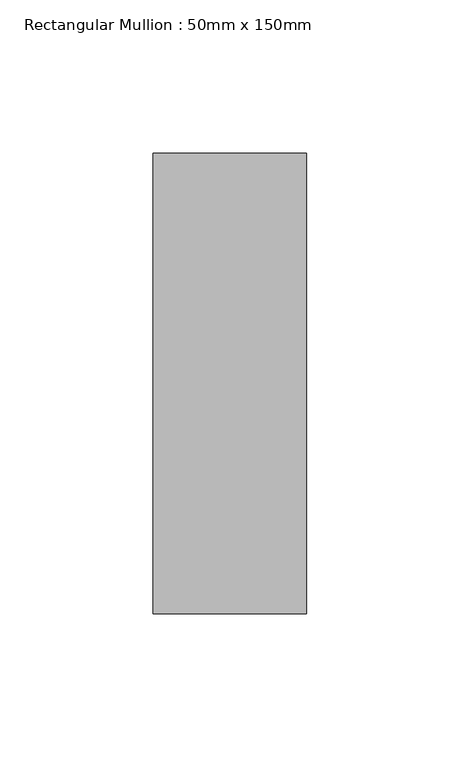
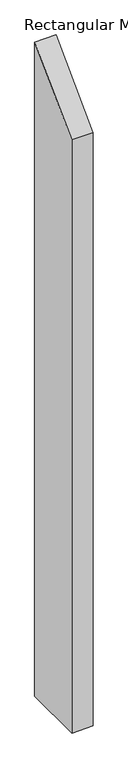
"""IFC4 building model written with IfcOpenShell, lengths in millimetres: member geometry, Rectangular Mullion : 50mm x 150mm."""

from ifc_helpers import new_model, si_unit, frame, origin, place, context, project, spatial, polyline, outline, extrude, source, transform, mapped, element, save


def rectangular_mullion_50mm_x_150mm_538b23cc(model_context):
    return source(origin(), model_context, "Body", "SweptSolid", [
        extrude(outline(polyline([(-75.0, -75.0), (75.0, 75.0), (75.0, -1538.6474098), (-75.0, -1538.6474098), (-75.0, -75.0)])), frame((-25.0, 0.0, 0.0), z_axis=(1.0, 0.0, 0.0), x_axis=(0.0, 1.0, 0.0)), (0.0, 0.0, 1.0), 50.0),
    ])


if __name__ == "__main__":
    model = new_model("IFC4")
    model_context = context("Model", 3, world=origin())
    ifc_project = project(units=[si_unit("LENGTHUNIT", "METRE", prefix="MILLI")], contexts=[model_context])
    site = spatial("IfcSite", under=ifc_project)
    building = spatial("IfcBuilding", under=site)
    placement = place(None, origin())
    rectangular_mullion_50mm_x_150mm_shape = rectangular_mullion_50mm_x_150mm_538b23cc(model_context)
    element("IfcMember", 1, ObjectType="Rectangular Mullion : 50mm x 150mm", at=placement, inside=building, context=model_context, shape_type="MappedRepresentation", body=[
        mapped(rectangular_mullion_50mm_x_150mm_shape, transform((0.0, 0.0, 0.0), x_axis=(1.0, 0.0, 0.0), y_axis=(0.0, 1.0, 0.0), z_axis=(0.0, 0.0, 1.0))),
    ])
    save(model, "model.ifc")

# Revit data of these elements
# Type "Rectangular Mullion : 50mm x 150mm"
#   built-in parameter 1007304 = 0.492126 (stored number, unit not read)
#   built-in parameter 1007301 = 0.082021 (stored number, unit not read)
#   built-in parameter 1007300 = 0.082021 (stored number, unit not read)
# Element 1 (IfcMember, "Rectangular Mullion : 50mm x 150mm")
#   Materials on its faces: "Aluminum"
# Materials
#   "Aluminum": class "Metal", colour RGB 244 244 244, transparency 0, Description = "Aluminum 6061", Cost = 0
